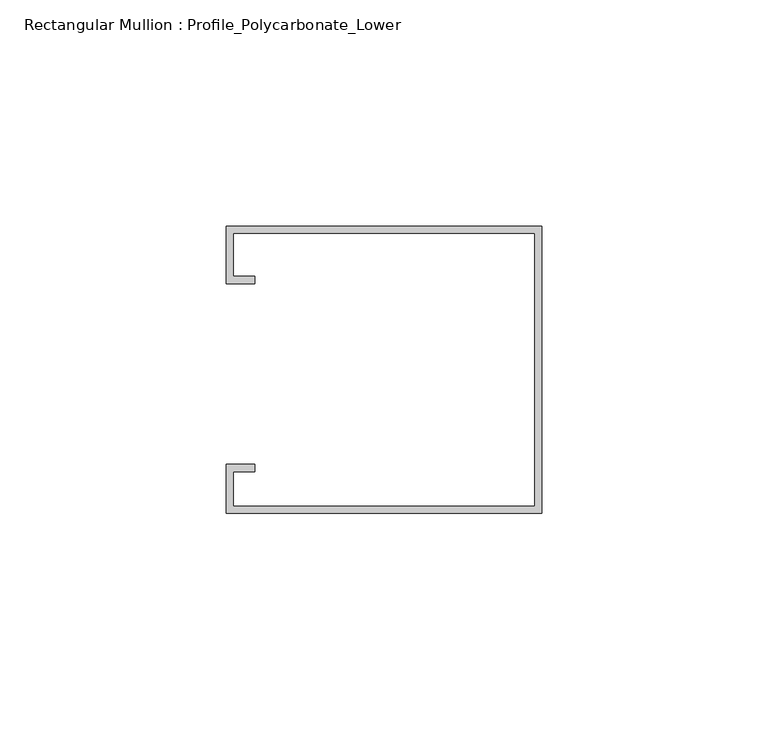
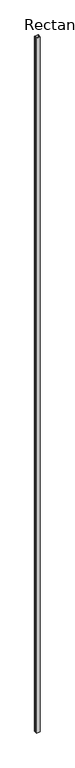
"""IFC4 building model written with IfcOpenShell, lengths in millimetres: member geometry, Rectangular Mullion : Profile_Polycarbonate_Lower."""

from ifc_helpers import new_model, si_unit, frame, origin, place, context, project, spatial, polyline, outline, extrude, source, transform, mapped, element, save


def rectangular_mullion_profile_polycarbonate_lower_e724aca0(model_context):
    return source(origin(), model_context, "Body", "SweptSolid", [
        extrude(outline(polyline([(0.0, 32.7), (0.0, -30.8), (-69.85, -30.8), (-69.85, -20.0), (-63.5, -20.0), (-63.5, -21.5875), (-68.2625, -21.5875), (-68.2625, -29.2125), (-1.5875, -29.2125), (-1.5875, 31.1125), (-68.2625, 31.1125), (-68.2625, 21.5875), (-63.5, 21.5875), (-63.5, 20.0), (-69.85, 20.0), (-69.85, 32.7), (0.0, 32.7)])), frame((0.0, 0.0, -14224.0), z_axis=(0.0, 0.0, 1.0), x_axis=(1.0, 0.0, 0.0)), (0.0, 0.0, 1.0), 14224.0),
    ])


if __name__ == "__main__":
    model = new_model("IFC4")
    model_context = context("Model", 3, world=origin())
    ifc_project = project(units=[si_unit("LENGTHUNIT", "METRE", prefix="MILLI")], contexts=[model_context])
    site = spatial("IfcSite", under=ifc_project)
    building = spatial("IfcBuilding", under=site)
    placement = place(None, origin())
    rectangular_mullion_profile_polycarbonate_lower_shape = rectangular_mullion_profile_polycarbonate_lower_e724aca0(model_context)
    element("IfcMember", 1, ObjectType="Rectangular Mullion : Profile_Polycarbonate_Lower", at=placement, inside=building, context=model_context, shape_type="MappedRepresentation", body=[
        mapped(rectangular_mullion_profile_polycarbonate_lower_shape, transform((0.0, 0.0, 0.0), x_axis=(1.0, 0.0, 0.0), y_axis=(0.0, 1.0, 0.0), z_axis=(0.0, 0.0, 1.0))),
    ])
    save(model, "model.ifc")

# Revit data of these elements
# Type "Rectangular Mullion : Profile_Polycarbonate_Lower"
#   built-in parameter 1007322 = 0.208333 (stored number, unit not read)
#   built-in parameter 1007321 = 0 (stored number, unit not read)
#   built-in parameter 1007320 = 0.00520833 (stored number, unit not read)
# Element 1 (IfcMember, "Rectangular Mullion : Profile_Polycarbonate_Lower")
#   Materials on its faces: "Aluminum"
# Materials
#   "Aluminum": class "Metal", colour RGB 244 244 244, transparency 0, Description = "Aluminum 6061", Cost = 0
